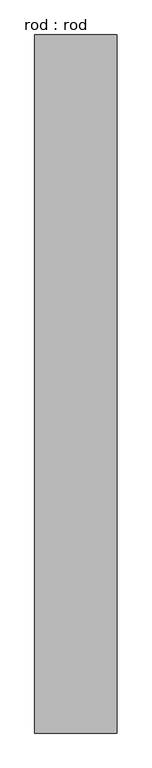
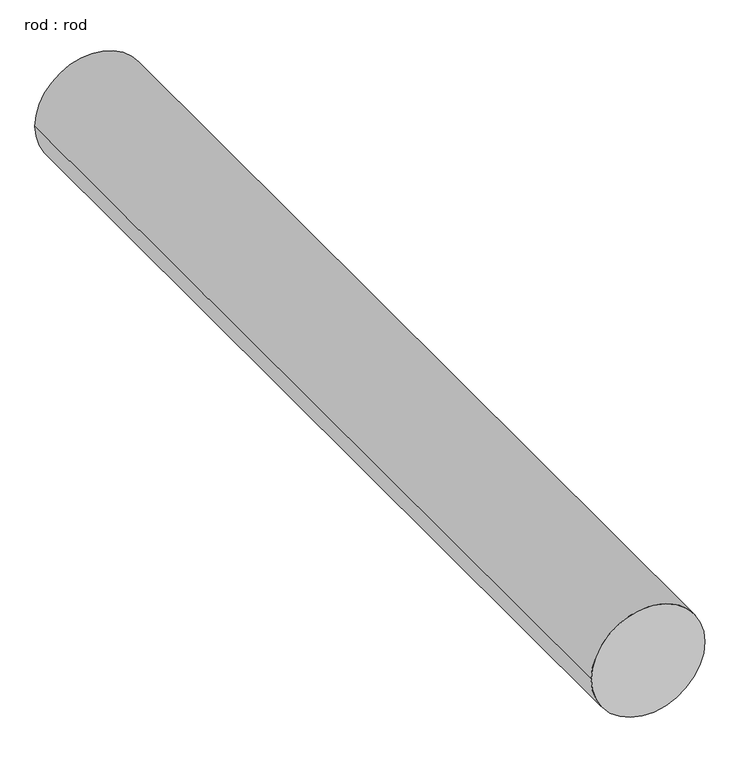
"""IFC4 building model written with IfcOpenShell, lengths in millimetres: proxy geometry, rod : rod."""

from ifc_helpers import new_model, si_unit, point, frame, frame_2d, origin, place, context, project, spatial, circle_curve, trimmed, segment, composite_curve, outline, extrude, source, transform, mapped, element, save


def rod_rod_d7f1f69e(model_context):
    return source(origin(), model_context, "Body", "SweptSolid", [
        extrude(outline(composite_curve([segment(trimmed(circle_curve(frame_2d((0.0108462, 0.0)), 200.0), [point((0.0108462, 200.0))], [point((0.0108462, -200.0))], False, "CARTESIAN"), True, "CONTINUOUS"), segment(trimmed(circle_curve(frame_2d((0.0108462, 0.0)), 200.0), [point((0.0108462, -200.0))], [point((0.0108462, 200.0))], False, "CARTESIAN"), True, "CONTINUOUS")], self_intersect=False)), frame((0.0, 2394.5143296, 0.0), z_axis=(0.0, 1.0, 0.0), x_axis=(0.0, 0.0, 1.0)), (0.0, 0.0, 1.0), 3396.4285714),
    ])


if __name__ == "__main__":
    model = new_model("IFC4")
    model_context = context("Model", 3, world=origin())
    ifc_project = project(units=[si_unit("LENGTHUNIT", "METRE", prefix="MILLI")], contexts=[model_context])
    site = spatial("IfcSite", under=ifc_project)
    building = spatial("IfcBuilding", under=site)
    placement = place(None, origin())
    rod_rod_shape = rod_rod_d7f1f69e(model_context)
    element("IfcBuildingElementProxy", 1, Name="rod : rod", ObjectType="rod : rod", at=placement, inside=building, context=model_context, shape_type="MappedRepresentation", body=[
        mapped(rod_rod_shape, transform((0.0, 0.0, 0.0), x_axis=(1.0, 0.0, 0.0), y_axis=(0.0, 1.0, 0.0), z_axis=(0.0, 0.0, 1.0))),
    ])
    save(model, "model.ifc")

# Revit data of these elements
# Type "rod : rod"
#   Default Elevation = 0
